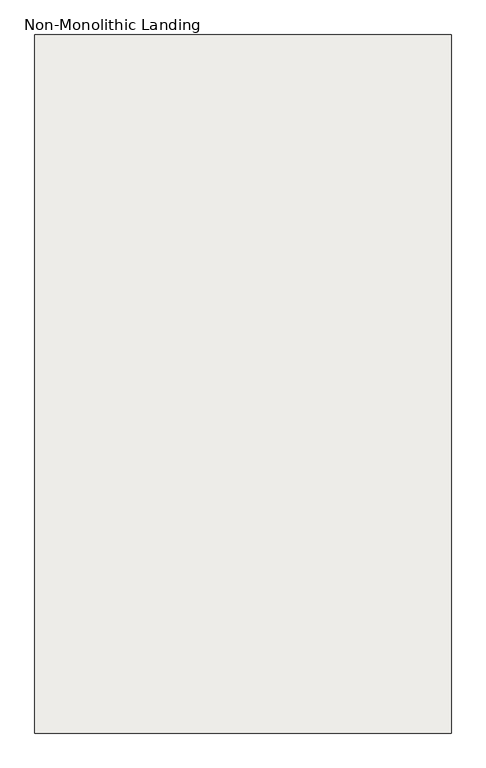
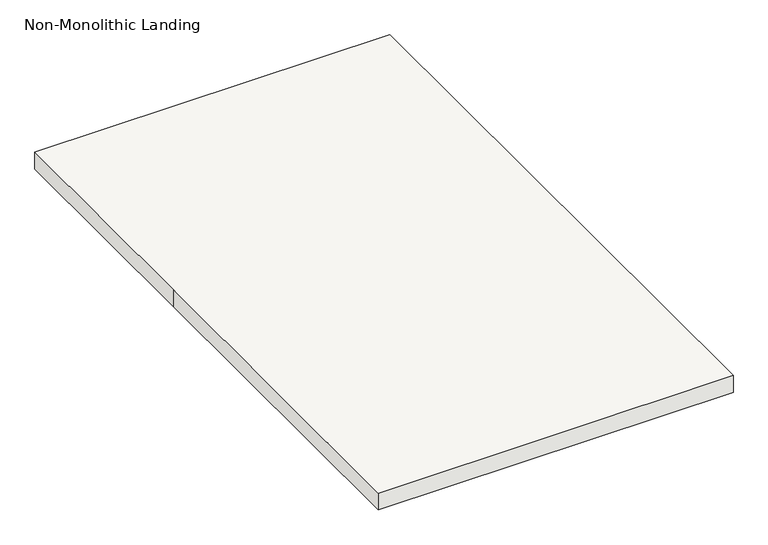
"""IFC4 building model written with IfcOpenShell, lengths in millimetres: slab geometry, Non-Monolithic Landing."""

import ifcopenshell
import ifcopenshell.guid

model = None  # the IFC model being written
_history = None  # IfcOwnerHistory: only IFC2X3 demands one
_inside = {}  # id of a spatial element -> (the spatial element, [elements in it])
_under = {}  # id of a project, library or spatial element -> (it, [spatial elements below it])
_declared = {}  # id of a project -> (the project, [libraries it declares])
_typed = {}  # id of a type object -> (the type object, [elements of that type])
_made_of = {}  # id of a material, layer set ... -> (it, [elements and type objects made of it])


def new_model(schema):
    """Start an empty IFC model of exactly this schema.

    Asked for "IFC4X3", IfcOpenShell would pick the latest addendum, in which some entities
    have other attributes; the version numbers below select the first issue.
    IFC2X3 requires an IfcOwnerHistory on every rooted entity: one is made here for all.
    """
    global model, _history
    if schema == "IFC4X3":
        model = ifcopenshell.file(schema_version=(4, 3, 0, 0))
    else:
        model = ifcopenshell.file(schema=schema)
    _inside.clear()
    _under.clear()
    _declared.clear()
    _typed.clear()
    _made_of.clear()
    _history = None
    if model.schema == "IFC2X3":
        org = make("IfcOrganization", Name="unknown")
        user = make(
            "IfcPersonAndOrganization",
            ThePerson=make("IfcPerson", FamilyName="unknown"),
            TheOrganization=org,
        )
        app = make(
            "IfcApplication",
            ApplicationDeveloper=org,
            Version="unknown",
            ApplicationFullName="unknown",
            ApplicationIdentifier="unknown",
        )
        _history = make(
            "IfcOwnerHistory",
            OwningUser=user,
            OwningApplication=app,
            ChangeAction="ADDED",
            CreationDate=0,
        )
    return model


def make(cls, **values):
    """One entity of the class cls with the attributes given. An attribute that is None is left unset."""
    return model.create_entity(
        cls, **{name: value for name, value in values.items() if value is not None}
    )


def rooted(cls, **values):
    """An entity with a GlobalId (a new one), such as an element, a storey or a relation."""
    return make(cls, GlobalId=ifcopenshell.guid.new(), OwnerHistory=_history, **values)


def si_unit(unit_type, name, prefix=None):
    """IfcSIUnit, for example si_unit("LENGTHUNIT", "METRE", prefix="MILLI")."""
    return make("IfcSIUnit", UnitType=unit_type, Prefix=prefix, Name=name)


def assignment(units):
    """IfcUnitAssignment: the units of a project."""
    return None if units is None else make("IfcUnitAssignment", Units=units)


def point(xyz):
    """IfcCartesianPoint."""
    return None if xyz is None else make("IfcCartesianPoint", Coordinates=xyz)


def direction(xyz):
    """IfcDirection."""
    return None if xyz is None else make("IfcDirection", DirectionRatios=xyz)


def frame(location, z_axis=None, x_axis=None):
    """IfcAxis2Placement3D, a coordinate frame: its origin and axes. An axis left out is left unset."""
    return make(
        "IfcAxis2Placement3D",
        Location=point(location),
        Axis=direction(z_axis),
        RefDirection=direction(x_axis),
    )


def origin():
    """The frame at (0, 0, 0) with its axes left unset."""
    return frame((0.0, 0.0, 0.0))


def place(relative_to, where):
    """IfcLocalPlacement: puts the frame where relative to a parent placement (None: the world)."""
    return make(
        "IfcLocalPlacement", PlacementRelTo=relative_to, RelativePlacement=where
    )


def context(
    kind, dimensions, precision=None, world=None, true_north=None, identifier=None
):
    """IfcGeometricRepresentationContext, for example the 3D "Model" context."""
    return make(
        "IfcGeometricRepresentationContext",
        ContextIdentifier=identifier,
        ContextType=kind,
        CoordinateSpaceDimension=dimensions,
        Precision=precision,
        WorldCoordinateSystem=world,
        TrueNorth=true_north,
    )


def project(units=None, contexts=None):
    """IfcProject with its units and contexts."""
    return rooted(
        "IfcProject",
        Name="project",
        RepresentationContexts=contexts,
        UnitsInContext=assignment(units),
    )


def spatial(cls, under=None, at=None, **own):
    """A site, building, storey or space (cls), placed at a placement, below another one or the project."""
    s = rooted(cls, ObjectPlacement=at, **own)
    if under is not None:
        _under.setdefault(under.id(), (under, []))[1].append(s)
    return s


def polyline(points):
    """IfcPolyline through the points."""
    return make("IfcPolyline", Points=[point(p) for p in points])


def outline(outer, holes=None, kind="AREA"):
    """IfcArbitraryClosedProfileDef: a profile drawn as a closed curve; with holes, ...WithVoids."""
    if holes is None:
        return make("IfcArbitraryClosedProfileDef", ProfileType=kind, OuterCurve=outer)
    return make(
        "IfcArbitraryProfileDefWithVoids",
        ProfileType=kind,
        OuterCurve=outer,
        InnerCurves=holes,
    )


def extrude(swept, where, along, depth):
    """IfcExtrudedAreaSolid: the profile swept, set in the frame where, extruded along a direction by depth."""
    return make(
        "IfcExtrudedAreaSolid",
        SweptArea=swept,
        Position=where,
        ExtrudedDirection=direction(along),
        Depth=depth,
    )


def shape(context_of_items, identifier, shape_type, items):
    """IfcShapeRepresentation: the items that make up one representation, for example the "Body"."""
    return make(
        "IfcShapeRepresentation",
        ContextOfItems=context_of_items,
        RepresentationIdentifier=identifier,
        RepresentationType=shape_type,
        Items=items,
    )


def source(mapping_origin, context_of_items, identifier, shape_type, items):
    """IfcRepresentationMap: a shape defined once, which mapped items show again and again."""
    return make(
        "IfcRepresentationMap",
        MappingOrigin=mapping_origin,
        MappedRepresentation=shape(context_of_items, identifier, shape_type, items),
    )


def transform(
    local_origin,
    x_axis=None,
    y_axis=None,
    z_axis=None,
    scale=None,
    scale2=None,
    scale3=None,
    uniform=True,
):
    """IfcCartesianTransformationOperator3D, or its non-uniform kind. x_axis, y_axis, z_axis: its Axis1, 2, 3."""
    if uniform:
        return make(
            "IfcCartesianTransformationOperator3D",
            Axis1=direction(x_axis),
            Axis2=direction(y_axis),
            LocalOrigin=point(local_origin),
            Scale=scale,
            Axis3=direction(z_axis),
        )
    return make(
        "IfcCartesianTransformationOperator3DnonUniform",
        Axis1=direction(x_axis),
        Axis2=direction(y_axis),
        LocalOrigin=point(local_origin),
        Scale=scale,
        Axis3=direction(z_axis),
        Scale2=scale2,
        Scale3=scale3,
    )


def mapped(mapping_source, mapping_target):
    """IfcMappedItem: shows the shape of a source again, moved by a transform."""
    return make(
        "IfcMappedItem", MappingSource=mapping_source, MappingTarget=mapping_target
    )


def made_of(thing, what):
    """Note that an element or type object is made of a material, layer set ...; save() writes the relation."""
    if what is not None:
        _made_of.setdefault(what.id(), (what, []))[1].append(thing)
    return thing


def element(
    cls,
    number,
    at=None,
    inside=None,
    cuts=None,
    type_object=None,
    material=None,
    context=None,
    identifier="Body",
    shape_type=None,
    held_by="IfcProductDefinitionShape",
    body=None,
    shapes=None,
    **own,
):
    """One element of the class cls, such as IfcWall. Its Tag is "e" and its number.

    at: its placement. inside: the storey or other place that contains it. cuts: it is an
    opening in that element (IfcRelVoidsElement). A single representation is given by context,
    identifier, shape_type and body (its items); several are given by shapes. held_by: the class
    of the entity that holds the representations. save() writes the other relations.
    """
    e = rooted(cls, Tag="e%d" % number, ObjectPlacement=at, **own)
    if body is not None:
        shapes = [shape(context, identifier, shape_type, body)]
    if shapes is not None:
        e.Representation = make(held_by, Representations=shapes)
    if inside is not None:
        _inside.setdefault(inside.id(), (inside, []))[1].append(e)
    if cuts is not None:
        rooted(
            "IfcRelVoidsElement", RelatingBuildingElement=cuts, RelatedOpeningElement=e
        )
    if type_object is not None:
        _typed.setdefault(type_object.id(), (type_object, []))[1].append(e)
    return made_of(e, material)


def aggregate(whole, parts):
    """IfcRelAggregates: a whole, such as a stair, and the parts it consists of."""
    return rooted("IfcRelAggregates", RelatingObject=whole, RelatedObjects=parts)


def save(model, path):
    """Write the relations noted so far, then the file.

    IfcRelAggregates (storeys below a building ...), IfcRelContainedInSpatialStructure (elements
    in a storey), IfcRelDefinesByType, IfcRelAssociatesMaterial and IfcRelDeclares: one each for
    every whole, place, type object, material and project.
    """
    for whole, parts in _under.values():
        aggregate(whole, parts)
    for where, things in _inside.values():
        rooted(
            "IfcRelContainedInSpatialStructure",
            RelatedElements=things,
            RelatingStructure=where,
        )
    for kind, things in _typed.values():
        rooted("IfcRelDefinesByType", RelatedObjects=things, RelatingType=kind)
    for what, things in _made_of.values():
        rooted("IfcRelAssociatesMaterial", RelatedObjects=things, RelatingMaterial=what)
    for by, libraries in _declared.values():
        rooted("IfcRelDeclares", RelatingContext=by, RelatedDefinitions=libraries)
    model.write(path)


def non_monolithic_landing_293fa1f8(model_context):
    return source(origin(), model_context, "Body", "SweptSolid", [
        extrude(outline(polyline([(21549.836337, -2576.2808257), (21549.836337, -1900.524372), (22549.836337, -1900.524372), (22549.836337, -3576.2808257), (21549.836337, -3576.2808257), (21549.836337, -2576.2808257)])), frame((0.0, 0.0, 1859.0909091), z_axis=(0.0, 0.0, 1.0), x_axis=(1.0, 0.0, 0.0)), (0.0, 0.0, 1.0), 50.0),
    ])


if __name__ == "__main__":
    model = new_model("IFC4")
    model_context = context("Model", 3, world=origin())
    ifc_project = project(units=[si_unit("LENGTHUNIT", "METRE", prefix="MILLI")], contexts=[model_context])
    site = spatial("IfcSite", under=ifc_project)
    building = spatial("IfcBuilding", under=site)
    placement = place(None, origin())
    non_monolithic_landing_shape = non_monolithic_landing_293fa1f8(model_context)
    element("IfcSlab", 1, ObjectType="Non-Monolithic Landing", at=placement, inside=building, context=model_context, shape_type="MappedRepresentation", body=[
        mapped(non_monolithic_landing_shape, transform((0.0, 0.0, 0.0), x_axis=(1.0, 0.0, 0.0), y_axis=(0.0, 1.0, 0.0), z_axis=(0.0, 0.0, 1.0))),
    ])
    save(model, "model.ifc")
